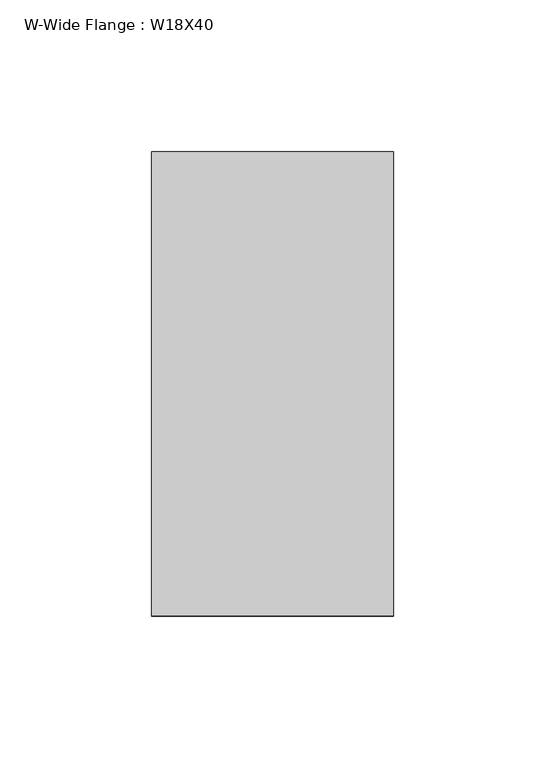
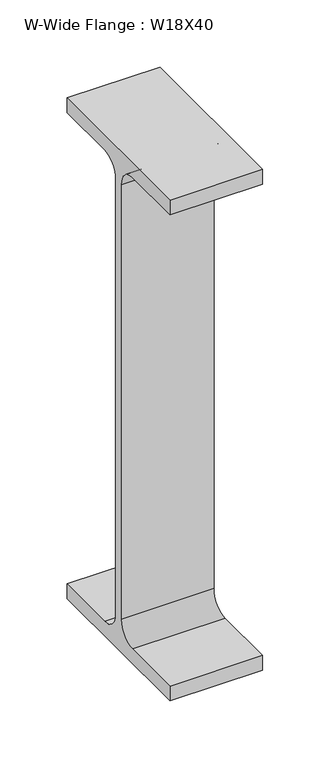
"""IFC4 building model written with IfcOpenShell, lengths in millimetres: beam geometry, W-Wide Flange : W18X40."""

from ifc_helpers import new_model, si_unit, point, frame, frame_2d, origin, place, context, project, spatial, polyline, circle_curve, trimmed, segment, composite_curve, outline, extrude, source, transform, mapped, element, save


def w_wide_flange_w18x40_5d36b511(model_context):
    return source(origin(), model_context, "Body", "SweptSolid", [
        extrude(outline(composite_curve([segment(polyline([(76.454, -213.995), (76.454, -227.33), (-76.454, -227.33), (-76.454, -213.995), (-20.828, -213.995)]), True, "CONTINUOUS"), segment(trimmed(circle_curve(frame_2d((-20.828, -197.1675)), 16.8275), [point((-20.828, -213.995))], [point((-4.0005, -197.1675))], True, "CARTESIAN"), True, "CONTINUOUS"), segment(polyline([(-4.0005, -197.1675), (-4.0005, 197.1675)]), True, "CONTINUOUS"), segment(trimmed(circle_curve(frame_2d((-20.828, 197.1675)), 16.8275), [point((-4.0005, 197.1675))], [point((-20.828, 213.995))], True, "CARTESIAN"), True, "CONTINUOUS"), segment(polyline([(-20.828, 213.995), (-76.454, 213.995), (-76.454, 227.33), (76.454, 227.33), (76.454, 213.995), (20.828, 213.995)]), True, "CONTINUOUS"), segment(trimmed(circle_curve(frame_2d((20.828, 197.1675)), 16.8275), [point((20.828, 213.995))], [point((4.0005, 197.1675))], True, "CARTESIAN"), True, "CONTINUOUS"), segment(polyline([(4.0005, 197.1675), (4.0005, -197.1675)]), True, "CONTINUOUS"), segment(trimmed(circle_curve(frame_2d((20.828, -197.1675)), 16.8275), [point((4.0005, -197.1675))], [point((20.828, -213.995))], True, "CARTESIAN"), True, "CONTINUOUS"), segment(polyline([(20.828, -213.995), (76.454, -213.995)]), True, "CONTINUOUS")], self_intersect=False)), frame((-68.2625, 0.0, 0.0), z_axis=(1.0, 0.0, 0.0), x_axis=(0.0, 1.0, 0.0)), (0.0, 0.0, 1.0), 79.6925),
    ])


if __name__ == "__main__":
    model = new_model("IFC4")
    model_context = context("Model", 3, world=origin())
    ifc_project = project(units=[si_unit("LENGTHUNIT", "METRE", prefix="MILLI")], contexts=[model_context])
    site = spatial("IfcSite", under=ifc_project)
    building = spatial("IfcBuilding", under=site)
    placement = place(None, origin())
    w_wide_flange_w18x40_shape = w_wide_flange_w18x40_5d36b511(model_context)
    element("IfcBeam", 1, ObjectType="W-Wide Flange : W18X40", at=placement, inside=building, context=model_context, shape_type="MappedRepresentation", body=[
        mapped(w_wide_flange_w18x40_shape, transform((0.0, 0.0, 0.0), x_axis=(1.0, 0.0, 0.0), y_axis=(0.0, 1.0, 0.0), z_axis=(0.0, 0.0, 1.0))),
    ])
    save(model, "model.ifc")

# Revit data of these elements
# Type "W-Wide Flange : W18X40"
#   Assembly Code = "B10"
#   W = 40
#   Length [instance default] = 5' - 0"
#   bf = 0' - 6.02"
#   d = 1' - 5.9"
#   k = 0' - 1 3/16"
#   k2 = 0' - 0.6625"
#   tf = 0' - 0.525"
#   tw = 0' - 0.315"
#   A = 0.0819444 SF
#   Structural Material [instance default] = Steel ASTM A992
# Element 1 (IfcBeam, "W-Wide Flange : W18X40")
#   Materials on its faces: "Steel ASTM A992"
# Materials
#   "Steel ASTM A992": class "Metal", colour RGB 199 199 199, transparency 0, Description = "Structural steel 50ksi", Cost = 0
